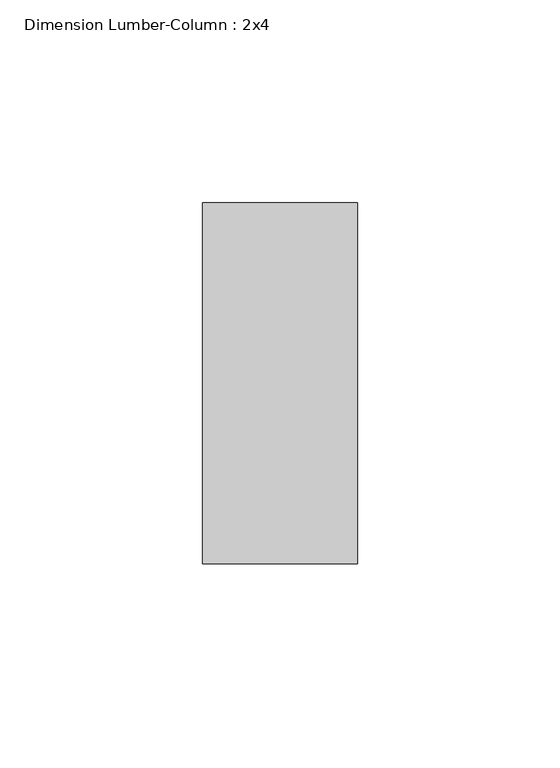
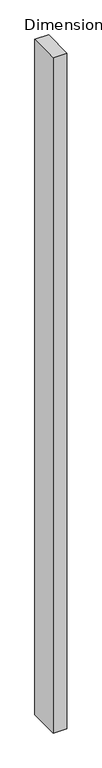
"""IFC4 building model written with IfcOpenShell, lengths in millimetres: column geometry, Dimension Lumber-Column : 2x4."""

from ifc_helpers import new_model, si_unit, frame, origin, place, context, project, spatial, polyline, outline, extrude, source, transform, mapped, element, save


def dimension_lumber_column_2x4_e13b243c(model_context):
    return source(origin(), model_context, "Body", "SweptSolid", [
        extrude(outline(polyline([(19.05, -44.45), (-19.05, -44.45), (-19.05, 44.45), (19.05, 44.45), (19.05, -44.45)])), frame((0.0, 0.0, 56.35625), z_axis=(0.0, 0.0, 1.0), x_axis=(1.0, 0.0, 0.0)), (0.0, 0.0, 1.0), 1999.853125),
    ])


if __name__ == "__main__":
    model = new_model("IFC4")
    model_context = context("Model", 3, world=origin())
    ifc_project = project(units=[si_unit("LENGTHUNIT", "METRE", prefix="MILLI")], contexts=[model_context])
    site = spatial("IfcSite", under=ifc_project)
    building = spatial("IfcBuilding", under=site)
    placement = place(None, origin())
    dimension_lumber_column_2x4_shape = dimension_lumber_column_2x4_e13b243c(model_context)
    element("IfcColumn", 1, ObjectType="Dimension Lumber-Column : 2x4", at=placement, inside=building, context=model_context, shape_type="MappedRepresentation", body=[
        mapped(dimension_lumber_column_2x4_shape, transform((0.0, 0.0, 0.0), x_axis=(1.0, 0.0, 0.0), y_axis=(0.0, 1.0, 0.0), z_axis=(0.0, 0.0, 1.0))),
    ])
    save(model, "model.ifc")

# Revit data of these elements
# Type "Dimension Lumber-Column : 2x4"
#   Int Type = "Interior"
#   Assembly Code = "B10"
#   Cost = 8.05
#   A = 0.0364583 SF
#   b = 0' - 1 1/2"
#   d = 0' - 3 1/2"
#   Structural Material [instance default] = Softwood, Lumber
# Element 1 (IfcColumn, "Dimension Lumber-Column : 2x4")
#   Structural Material = Douglas Fir #2
#   Materials on its faces: "Douglas Fir #2"
# Materials
#   "Softwood, Lumber": class "Wood", colour RGB 223 192 134, transparency 0, Description = "Pinus Echinata", Cost = 0
#   "Douglas Fir #2": class "Wood", colour RGB 223 192 134, transparency 0, Description = "Pinus Echinata", Cost = 0
